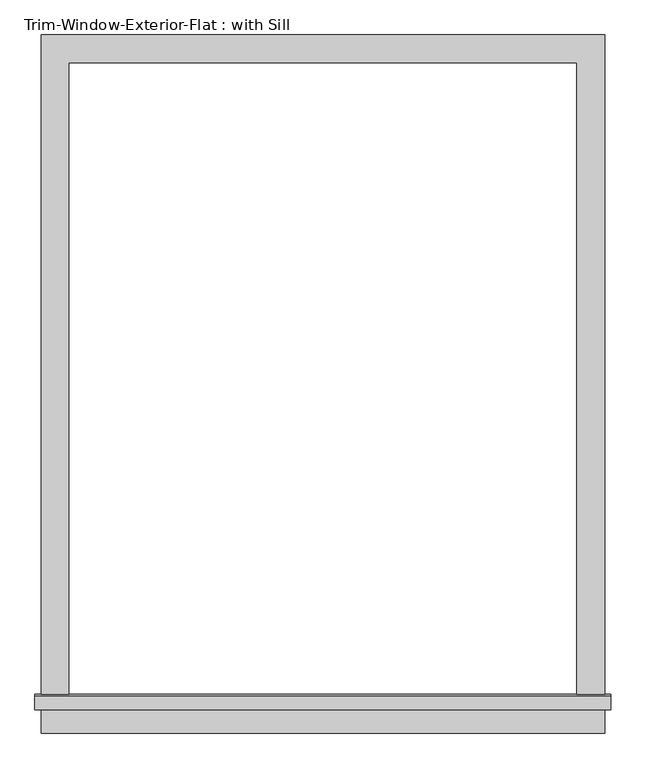
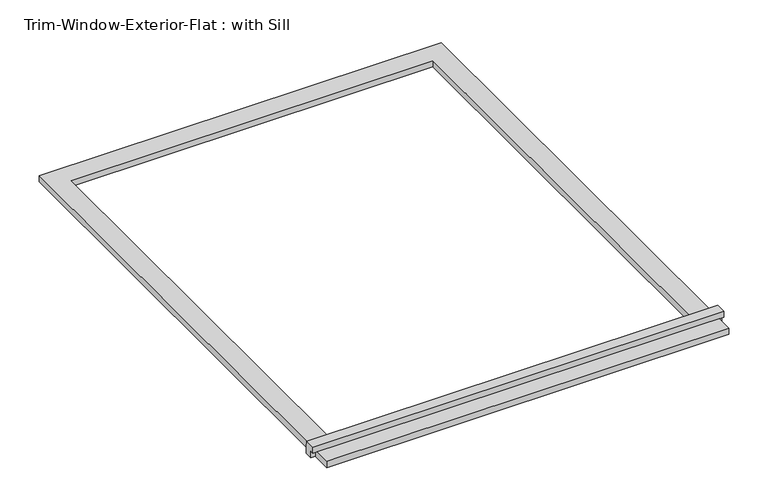
"""IFC4 building model written with IfcOpenShell, lengths in millimetres: proxy geometry, Trim-Window-Exterior-Flat : with Sill."""

import ifcopenshell
import ifcopenshell.guid

model = None  # the IFC model being written
_history = None  # IfcOwnerHistory: only IFC2X3 demands one
_inside = {}  # id of a spatial element -> (the spatial element, [elements in it])
_under = {}  # id of a project, library or spatial element -> (it, [spatial elements below it])
_declared = {}  # id of a project -> (the project, [libraries it declares])
_typed = {}  # id of a type object -> (the type object, [elements of that type])
_made_of = {}  # id of a material, layer set ... -> (it, [elements and type objects made of it])


def new_model(schema):
    """Start an empty IFC model of exactly this schema.

    Asked for "IFC4X3", IfcOpenShell would pick the latest addendum, in which some entities
    have other attributes; the version numbers below select the first issue.
    IFC2X3 requires an IfcOwnerHistory on every rooted entity: one is made here for all.
    """
    global model, _history
    if schema == "IFC4X3":
        model = ifcopenshell.file(schema_version=(4, 3, 0, 0))
    else:
        model = ifcopenshell.file(schema=schema)
    _inside.clear()
    _under.clear()
    _declared.clear()
    _typed.clear()
    _made_of.clear()
    _history = None
    if model.schema == "IFC2X3":
        org = make("IfcOrganization", Name="unknown")
        user = make(
            "IfcPersonAndOrganization",
            ThePerson=make("IfcPerson", FamilyName="unknown"),
            TheOrganization=org,
        )
        app = make(
            "IfcApplication",
            ApplicationDeveloper=org,
            Version="unknown",
            ApplicationFullName="unknown",
            ApplicationIdentifier="unknown",
        )
        _history = make(
            "IfcOwnerHistory",
            OwningUser=user,
            OwningApplication=app,
            ChangeAction="ADDED",
            CreationDate=0,
        )
    return model


def make(cls, **values):
    """One entity of the class cls with the attributes given. An attribute that is None is left unset."""
    return model.create_entity(
        cls, **{name: value for name, value in values.items() if value is not None}
    )


def rooted(cls, **values):
    """An entity with a GlobalId (a new one), such as an element, a storey or a relation."""
    return make(cls, GlobalId=ifcopenshell.guid.new(), OwnerHistory=_history, **values)


def si_unit(unit_type, name, prefix=None):
    """IfcSIUnit, for example si_unit("LENGTHUNIT", "METRE", prefix="MILLI")."""
    return make("IfcSIUnit", UnitType=unit_type, Prefix=prefix, Name=name)


def assignment(units):
    """IfcUnitAssignment: the units of a project."""
    return None if units is None else make("IfcUnitAssignment", Units=units)


def point(xyz):
    """IfcCartesianPoint."""
    return None if xyz is None else make("IfcCartesianPoint", Coordinates=xyz)


def direction(xyz):
    """IfcDirection."""
    return None if xyz is None else make("IfcDirection", DirectionRatios=xyz)


def frame(location, z_axis=None, x_axis=None):
    """IfcAxis2Placement3D, a coordinate frame: its origin and axes. An axis left out is left unset."""
    return make(
        "IfcAxis2Placement3D",
        Location=point(location),
        Axis=direction(z_axis),
        RefDirection=direction(x_axis),
    )


def origin():
    """The frame at (0, 0, 0) with its axes left unset."""
    return frame((0.0, 0.0, 0.0))


def origin_with_axes():
    """The frame at (0, 0, 0) with the z axis (0, 0, 1) and the x axis (1, 0, 0) written out."""
    return frame((0.0, 0.0, 0.0), z_axis=(0.0, 0.0, 1.0), x_axis=(1.0, 0.0, 0.0))


def place(relative_to, where):
    """IfcLocalPlacement: puts the frame where relative to a parent placement (None: the world)."""
    return make(
        "IfcLocalPlacement", PlacementRelTo=relative_to, RelativePlacement=where
    )


def context(
    kind, dimensions, precision=None, world=None, true_north=None, identifier=None
):
    """IfcGeometricRepresentationContext, for example the 3D "Model" context."""
    return make(
        "IfcGeometricRepresentationContext",
        ContextIdentifier=identifier,
        ContextType=kind,
        CoordinateSpaceDimension=dimensions,
        Precision=precision,
        WorldCoordinateSystem=world,
        TrueNorth=true_north,
    )


def project(units=None, contexts=None):
    """IfcProject with its units and contexts."""
    return rooted(
        "IfcProject",
        Name="project",
        RepresentationContexts=contexts,
        UnitsInContext=assignment(units),
    )


def spatial(cls, under=None, at=None, **own):
    """A site, building, storey or space (cls), placed at a placement, below another one or the project."""
    s = rooted(cls, ObjectPlacement=at, **own)
    if under is not None:
        _under.setdefault(under.id(), (under, []))[1].append(s)
    return s


def polyline(points):
    """IfcPolyline through the points."""
    return make("IfcPolyline", Points=[point(p) for p in points])


def outline(outer, holes=None, kind="AREA"):
    """IfcArbitraryClosedProfileDef: a profile drawn as a closed curve; with holes, ...WithVoids."""
    if holes is None:
        return make("IfcArbitraryClosedProfileDef", ProfileType=kind, OuterCurve=outer)
    return make(
        "IfcArbitraryProfileDefWithVoids",
        ProfileType=kind,
        OuterCurve=outer,
        InnerCurves=holes,
    )


def extrude(swept, where, along, depth):
    """IfcExtrudedAreaSolid: the profile swept, set in the frame where, extruded along a direction by depth."""
    return make(
        "IfcExtrudedAreaSolid",
        SweptArea=swept,
        Position=where,
        ExtrudedDirection=direction(along),
        Depth=depth,
    )


def shape(context_of_items, identifier, shape_type, items):
    """IfcShapeRepresentation: the items that make up one representation, for example the "Body"."""
    return make(
        "IfcShapeRepresentation",
        ContextOfItems=context_of_items,
        RepresentationIdentifier=identifier,
        RepresentationType=shape_type,
        Items=items,
    )


def source(mapping_origin, context_of_items, identifier, shape_type, items):
    """IfcRepresentationMap: a shape defined once, which mapped items show again and again."""
    return make(
        "IfcRepresentationMap",
        MappingOrigin=mapping_origin,
        MappedRepresentation=shape(context_of_items, identifier, shape_type, items),
    )


def transform(
    local_origin,
    x_axis=None,
    y_axis=None,
    z_axis=None,
    scale=None,
    scale2=None,
    scale3=None,
    uniform=True,
):
    """IfcCartesianTransformationOperator3D, or its non-uniform kind. x_axis, y_axis, z_axis: its Axis1, 2, 3."""
    if uniform:
        return make(
            "IfcCartesianTransformationOperator3D",
            Axis1=direction(x_axis),
            Axis2=direction(y_axis),
            LocalOrigin=point(local_origin),
            Scale=scale,
            Axis3=direction(z_axis),
        )
    return make(
        "IfcCartesianTransformationOperator3DnonUniform",
        Axis1=direction(x_axis),
        Axis2=direction(y_axis),
        LocalOrigin=point(local_origin),
        Scale=scale,
        Axis3=direction(z_axis),
        Scale2=scale2,
        Scale3=scale3,
    )


def mapped(mapping_source, mapping_target):
    """IfcMappedItem: shows the shape of a source again, moved by a transform."""
    return make(
        "IfcMappedItem", MappingSource=mapping_source, MappingTarget=mapping_target
    )


def made_of(thing, what):
    """Note that an element or type object is made of a material, layer set ...; save() writes the relation."""
    if what is not None:
        _made_of.setdefault(what.id(), (what, []))[1].append(thing)
    return thing


def element(
    cls,
    number,
    at=None,
    inside=None,
    cuts=None,
    type_object=None,
    material=None,
    context=None,
    identifier="Body",
    shape_type=None,
    held_by="IfcProductDefinitionShape",
    body=None,
    shapes=None,
    **own,
):
    """One element of the class cls, such as IfcWall. Its Tag is "e" and its number.

    at: its placement. inside: the storey or other place that contains it. cuts: it is an
    opening in that element (IfcRelVoidsElement). A single representation is given by context,
    identifier, shape_type and body (its items); several are given by shapes. held_by: the class
    of the entity that holds the representations. save() writes the other relations.
    """
    e = rooted(cls, Tag="e%d" % number, ObjectPlacement=at, **own)
    if body is not None:
        shapes = [shape(context, identifier, shape_type, body)]
    if shapes is not None:
        e.Representation = make(held_by, Representations=shapes)
    if inside is not None:
        _inside.setdefault(inside.id(), (inside, []))[1].append(e)
    if cuts is not None:
        rooted(
            "IfcRelVoidsElement", RelatingBuildingElement=cuts, RelatedOpeningElement=e
        )
    if type_object is not None:
        _typed.setdefault(type_object.id(), (type_object, []))[1].append(e)
    return made_of(e, material)


def aggregate(whole, parts):
    """IfcRelAggregates: a whole, such as a stair, and the parts it consists of."""
    return rooted("IfcRelAggregates", RelatingObject=whole, RelatedObjects=parts)


def save(model, path):
    """Write the relations noted so far, then the file.

    IfcRelAggregates (storeys below a building ...), IfcRelContainedInSpatialStructure (elements
    in a storey), IfcRelDefinesByType, IfcRelAssociatesMaterial and IfcRelDeclares: one each for
    every whole, place, type object, material and project.
    """
    for whole, parts in _under.values():
        aggregate(whole, parts)
    for where, things in _inside.values():
        rooted(
            "IfcRelContainedInSpatialStructure",
            RelatedElements=things,
            RelatingStructure=where,
        )
    for kind, things in _typed.values():
        rooted("IfcRelDefinesByType", RelatedObjects=things, RelatingType=kind)
    for what, things in _made_of.values():
        rooted("IfcRelAssociatesMaterial", RelatedObjects=things, RelatingMaterial=what)
    for by, libraries in _declared.values():
        rooted("IfcRelDeclares", RelatingContext=by, RelatedDefinitions=libraries)
    model.write(path)


def trim_window_exterior_flat_with_sill_39d4c871(model_context):
    return source(origin(), model_context, "Body", "SweptSolid", [
        extrude(outline(polyline([(577.85, -1317.5823709), (577.85, -1374.7323709), (-577.85, -1374.7323709), (-577.85, -1317.5823709), (577.85, -1317.5823709)])), origin_with_axes(), (0.0, 0.0, 1.0), 19.05),
        extrude(outline(polyline([(-1327.15, 38.1), (-1297.8580645, 38.1), (-1295.4, 19.05), (-1295.4, 0.0), (-1317.5823709, 0.0), (-1317.5823709, 19.05), (-1327.15, 19.05), (-1327.15, 38.1)])), frame((-590.55, 0.0, 0.0), z_axis=(1.0, 0.0, 0.0), x_axis=(0.0, 1.0, 0.0)), (0.0, 0.0, 1.0), 1181.1),
        extrude(outline(polyline([(-577.85, 57.15), (577.85, 57.15), (577.85, -1295.4), (520.7, -1295.4), (520.7, 0.0), (-520.7, 0.0), (-520.7, -1295.4), (-577.85, -1295.4), (-577.85, 57.15)])), origin_with_axes(), (0.0, 0.0, 1.0), 19.05),
    ])


if __name__ == "__main__":
    model = new_model("IFC4")
    model_context = context("Model", 3, world=origin())
    ifc_project = project(units=[si_unit("LENGTHUNIT", "METRE", prefix="MILLI")], contexts=[model_context])
    site = spatial("IfcSite", under=ifc_project)
    building = spatial("IfcBuilding", under=site)
    placement = place(None, origin())
    trim_window_exterior_flat_with_sill_shape = trim_window_exterior_flat_with_sill_39d4c871(model_context)
    element("IfcBuildingElementProxy", 1, Name="Trim-Window-Exterior-Flat : with Sill", ObjectType="Trim-Window-Exterior-Flat : with Sill", at=placement, inside=building, context=model_context, shape_type="MappedRepresentation", body=[
        mapped(trim_window_exterior_flat_with_sill_shape, transform((0.0, 0.0, 0.0), x_axis=(1.0, 0.0, 0.0), y_axis=(0.0, 1.0, 0.0), z_axis=(0.0, 0.0, 1.0))),
    ])
    save(model, "model.ifc")

# Revit data of these elements
# Type "Trim-Window-Exterior-Flat : with Sill"
#   Trim Width = 0' - 2 1/4"
#   Trim Thickness_Picture Frame = 0' - 1 1/4"
#   Trim Thickness_with Sill = 0' - 0 3/4"
#   Sill Thickness = 0' - 1 1/4"
#   Opening Width [instance default] = 2' - 0"
#   Opening Height [instance default] = 3' - 0"
#   Default Elevation = 4' - 0"
#   Sill = yes
#   Picture Frame = no
#   Trim Material [instance default] = none
# Element 1 (IfcBuildingElementProxy, "Trim-Window-Exterior-Flat : with Sill")
#   Opening Width = 3' - 5"
#   Opening Height = 4' - 3"
#   Trim Material = Clad - White
#   Materials on its faces: "Clad - White"
# Materials
#   "Clad - White": class "Wood", colour RGB 242 242 238, transparency 0, Cost = 0
